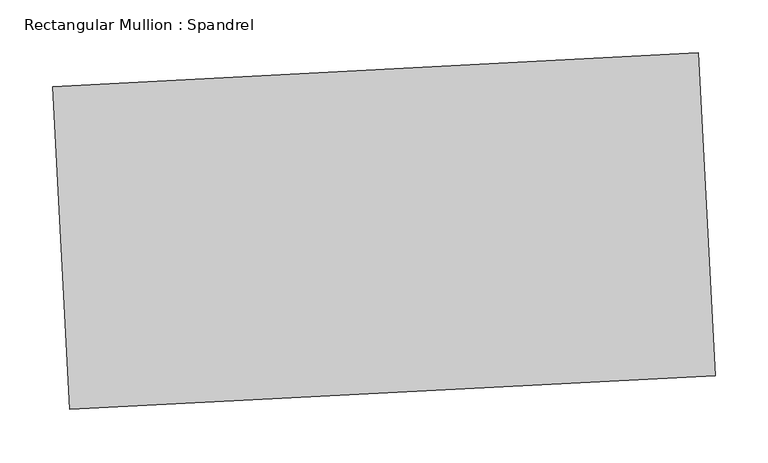
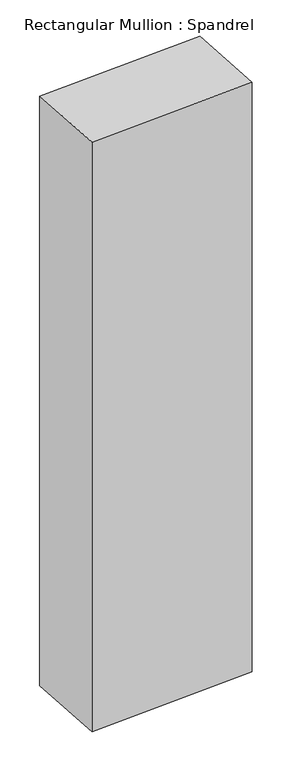
"""IFC4 building model written with IfcOpenShell, lengths in millimetres: member geometry, Rectangular Mullion : Spandrel."""

from ifc_helpers import new_model, si_unit, frame, origin, place, context, project, spatial, polyline, outline, extrude, source, transform, mapped, element, save


def rectangular_mullion_spandrel_c07370e7(model_context):
    return source(origin(), model_context, "Body", "SweptSolid", [
        extrude(outline(polyline([(-617.1582819, 136.2391416), (-8.3937175, 168.1431406), (7.5582819, -136.2391416), (-601.2062825, -168.1431406), (-617.1582819, 136.2391416)])), frame((0.0, 0.0, -2293.6958315), z_axis=(0.0, 0.0, 1.0), x_axis=(1.0, 0.0, 0.0)), (0.0, 0.0, 1.0), 2293.6958315),
    ])


if __name__ == "__main__":
    model = new_model("IFC4")
    model_context = context("Model", 3, world=origin())
    ifc_project = project(units=[si_unit("LENGTHUNIT", "METRE", prefix="MILLI")], contexts=[model_context])
    site = spatial("IfcSite", under=ifc_project)
    building = spatial("IfcBuilding", under=site)
    placement = place(None, origin())
    rectangular_mullion_spandrel_shape = rectangular_mullion_spandrel_c07370e7(model_context)
    element("IfcMember", 1, ObjectType="Rectangular Mullion : Spandrel", at=placement, inside=building, context=model_context, shape_type="MappedRepresentation", body=[
        mapped(rectangular_mullion_spandrel_shape, transform((0.0, 0.0, 0.0), x_axis=(1.0, 0.0, 0.0), y_axis=(0.0, 1.0, 0.0), z_axis=(0.0, 0.0, 1.0))),
    ])
    save(model, "model.ifc")

# Revit data of these elements
# Type "Rectangular Mullion : Spandrel"
#   built-in parameter 1007304 = 1 (stored number, unit not read)
#   built-in parameter 1007301 = 1 (stored number, unit not read)
#   built-in parameter 1007300 = 1 (stored number, unit not read)
# Element 1 (IfcMember, "Rectangular Mullion : Spandrel")
#   Materials on its faces: "Aluminum"
# Materials
#   "Aluminum": class "Metal", colour RGB 247 247 247, transparency 0, Description = "Aluminum 6061", Cost = 0
